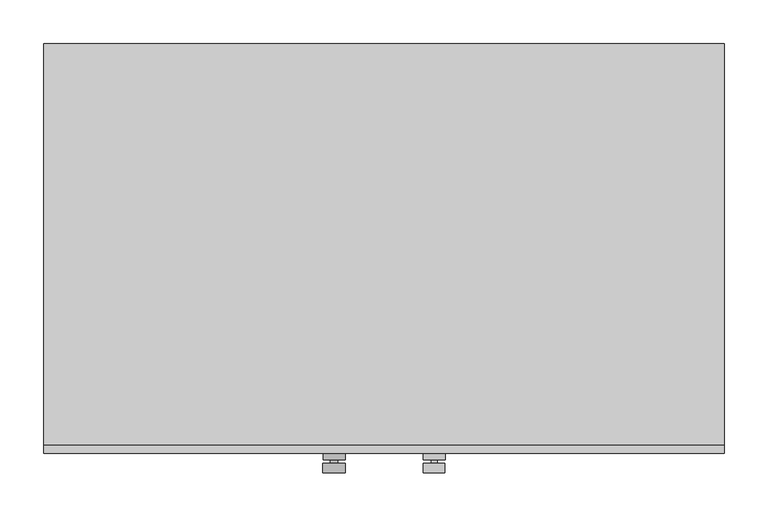
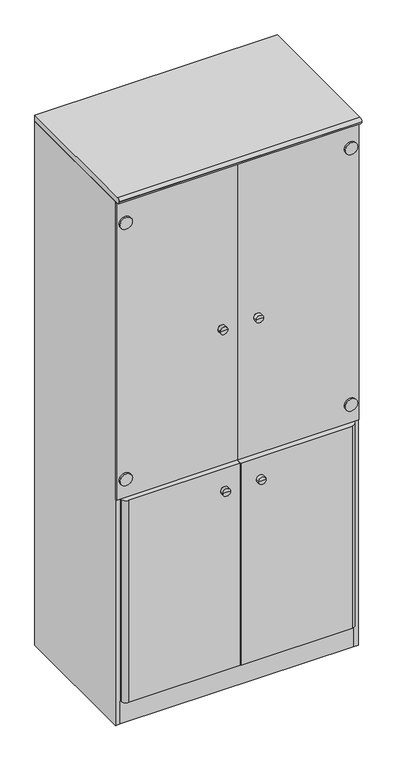
"""IFC4 building model written with IfcOpenShell, lengths in millimetres: furniture geometry, 书柜5 : W780*D450*H1800mm."""

import ifcopenshell
import ifcopenshell.guid

model = None  # the IFC model being written
_history = None  # IfcOwnerHistory: only IFC2X3 demands one
_inside = {}  # id of a spatial element -> (the spatial element, [elements in it])
_under = {}  # id of a project, library or spatial element -> (it, [spatial elements below it])
_declared = {}  # id of a project -> (the project, [libraries it declares])
_typed = {}  # id of a type object -> (the type object, [elements of that type])
_made_of = {}  # id of a material, layer set ... -> (it, [elements and type objects made of it])


def new_model(schema):
    """Start an empty IFC model of exactly this schema.

    Asked for "IFC4X3", IfcOpenShell would pick the latest addendum, in which some entities
    have other attributes; the version numbers below select the first issue.
    IFC2X3 requires an IfcOwnerHistory on every rooted entity: one is made here for all.
    """
    global model, _history
    if schema == "IFC4X3":
        model = ifcopenshell.file(schema_version=(4, 3, 0, 0))
    else:
        model = ifcopenshell.file(schema=schema)
    _inside.clear()
    _under.clear()
    _declared.clear()
    _typed.clear()
    _made_of.clear()
    _history = None
    if model.schema == "IFC2X3":
        org = make("IfcOrganization", Name="unknown")
        user = make(
            "IfcPersonAndOrganization",
            ThePerson=make("IfcPerson", FamilyName="unknown"),
            TheOrganization=org,
        )
        app = make(
            "IfcApplication",
            ApplicationDeveloper=org,
            Version="unknown",
            ApplicationFullName="unknown",
            ApplicationIdentifier="unknown",
        )
        _history = make(
            "IfcOwnerHistory",
            OwningUser=user,
            OwningApplication=app,
            ChangeAction="ADDED",
            CreationDate=0,
        )
    return model


def make(cls, **values):
    """One entity of the class cls with the attributes given. An attribute that is None is left unset."""
    return model.create_entity(
        cls, **{name: value for name, value in values.items() if value is not None}
    )


def rooted(cls, **values):
    """An entity with a GlobalId (a new one), such as an element, a storey or a relation."""
    return make(cls, GlobalId=ifcopenshell.guid.new(), OwnerHistory=_history, **values)


def si_unit(unit_type, name, prefix=None):
    """IfcSIUnit, for example si_unit("LENGTHUNIT", "METRE", prefix="MILLI")."""
    return make("IfcSIUnit", UnitType=unit_type, Prefix=prefix, Name=name)


def assignment(units):
    """IfcUnitAssignment: the units of a project."""
    return None if units is None else make("IfcUnitAssignment", Units=units)


def point(xyz):
    """IfcCartesianPoint."""
    return None if xyz is None else make("IfcCartesianPoint", Coordinates=xyz)


def direction(xyz):
    """IfcDirection."""
    return None if xyz is None else make("IfcDirection", DirectionRatios=xyz)


def frame(location, z_axis=None, x_axis=None):
    """IfcAxis2Placement3D, a coordinate frame: its origin and axes. An axis left out is left unset."""
    return make(
        "IfcAxis2Placement3D",
        Location=point(location),
        Axis=direction(z_axis),
        RefDirection=direction(x_axis),
    )


def frame_2d(location, x_axis=None):
    """IfcAxis2Placement2D, a coordinate frame in the plane: its origin and x axis."""
    return make(
        "IfcAxis2Placement2D", Location=point(location), RefDirection=direction(x_axis)
    )


def origin():
    """The frame at (0, 0, 0) with its axes left unset."""
    return frame((0.0, 0.0, 0.0))


def origin_with_axes():
    """The frame at (0, 0, 0) with the z axis (0, 0, 1) and the x axis (1, 0, 0) written out."""
    return frame((0.0, 0.0, 0.0), z_axis=(0.0, 0.0, 1.0), x_axis=(1.0, 0.0, 0.0))


def place(relative_to, where):
    """IfcLocalPlacement: puts the frame where relative to a parent placement (None: the world)."""
    return make(
        "IfcLocalPlacement", PlacementRelTo=relative_to, RelativePlacement=where
    )


def context(
    kind, dimensions, precision=None, world=None, true_north=None, identifier=None
):
    """IfcGeometricRepresentationContext, for example the 3D "Model" context."""
    return make(
        "IfcGeometricRepresentationContext",
        ContextIdentifier=identifier,
        ContextType=kind,
        CoordinateSpaceDimension=dimensions,
        Precision=precision,
        WorldCoordinateSystem=world,
        TrueNorth=true_north,
    )


def project(units=None, contexts=None):
    """IfcProject with its units and contexts."""
    return rooted(
        "IfcProject",
        Name="project",
        RepresentationContexts=contexts,
        UnitsInContext=assignment(units),
    )


def spatial(cls, under=None, at=None, **own):
    """A site, building, storey or space (cls), placed at a placement, below another one or the project."""
    s = rooted(cls, ObjectPlacement=at, **own)
    if under is not None:
        _under.setdefault(under.id(), (under, []))[1].append(s)
    return s


def polyline(points):
    """IfcPolyline through the points."""
    return make("IfcPolyline", Points=[point(p) for p in points])


def circle_curve(where, radius):
    """IfcCircle in the frame where."""
    return make("IfcCircle", Position=where, Radius=radius)


def trimmed(basis, trim1, trim2, sense, master):
    """IfcTrimmedCurve: the piece of a basis curve between two trims."""
    return make(
        "IfcTrimmedCurve",
        BasisCurve=basis,
        Trim1=trim1,
        Trim2=trim2,
        SenseAgreement=sense,
        MasterRepresentation=master,
    )


def segment(curve, same_sense, transition):
    """IfcCompositeCurveSegment."""
    return make(
        "IfcCompositeCurveSegment",
        Transition=transition,
        SameSense=same_sense,
        ParentCurve=curve,
    )


def composite_curve(segments, self_intersect=None):
    """IfcCompositeCurve: segments joined end to end."""
    return make("IfcCompositeCurve", Segments=segments, SelfIntersect=self_intersect)


def outline(outer, holes=None, kind="AREA"):
    """IfcArbitraryClosedProfileDef: a profile drawn as a closed curve; with holes, ...WithVoids."""
    if holes is None:
        return make("IfcArbitraryClosedProfileDef", ProfileType=kind, OuterCurve=outer)
    return make(
        "IfcArbitraryProfileDefWithVoids",
        ProfileType=kind,
        OuterCurve=outer,
        InnerCurves=holes,
    )


def extrude(swept, where, along, depth):
    """IfcExtrudedAreaSolid: the profile swept, set in the frame where, extruded along a direction by depth."""
    return make(
        "IfcExtrudedAreaSolid",
        SweptArea=swept,
        Position=where,
        ExtrudedDirection=direction(along),
        Depth=depth,
    )


def shape(context_of_items, identifier, shape_type, items):
    """IfcShapeRepresentation: the items that make up one representation, for example the "Body"."""
    return make(
        "IfcShapeRepresentation",
        ContextOfItems=context_of_items,
        RepresentationIdentifier=identifier,
        RepresentationType=shape_type,
        Items=items,
    )


def source(mapping_origin, context_of_items, identifier, shape_type, items):
    """IfcRepresentationMap: a shape defined once, which mapped items show again and again."""
    return make(
        "IfcRepresentationMap",
        MappingOrigin=mapping_origin,
        MappedRepresentation=shape(context_of_items, identifier, shape_type, items),
    )


def transform(
    local_origin,
    x_axis=None,
    y_axis=None,
    z_axis=None,
    scale=None,
    scale2=None,
    scale3=None,
    uniform=True,
):
    """IfcCartesianTransformationOperator3D, or its non-uniform kind. x_axis, y_axis, z_axis: its Axis1, 2, 3."""
    if uniform:
        return make(
            "IfcCartesianTransformationOperator3D",
            Axis1=direction(x_axis),
            Axis2=direction(y_axis),
            LocalOrigin=point(local_origin),
            Scale=scale,
            Axis3=direction(z_axis),
        )
    return make(
        "IfcCartesianTransformationOperator3DnonUniform",
        Axis1=direction(x_axis),
        Axis2=direction(y_axis),
        LocalOrigin=point(local_origin),
        Scale=scale,
        Axis3=direction(z_axis),
        Scale2=scale2,
        Scale3=scale3,
    )


def mapped(mapping_source, mapping_target):
    """IfcMappedItem: shows the shape of a source again, moved by a transform."""
    return make(
        "IfcMappedItem", MappingSource=mapping_source, MappingTarget=mapping_target
    )


def made_of(thing, what):
    """Note that an element or type object is made of a material, layer set ...; save() writes the relation."""
    if what is not None:
        _made_of.setdefault(what.id(), (what, []))[1].append(thing)
    return thing


def element(
    cls,
    number,
    at=None,
    inside=None,
    cuts=None,
    type_object=None,
    material=None,
    context=None,
    identifier="Body",
    shape_type=None,
    held_by="IfcProductDefinitionShape",
    body=None,
    shapes=None,
    **own,
):
    """One element of the class cls, such as IfcWall. Its Tag is "e" and its number.

    at: its placement. inside: the storey or other place that contains it. cuts: it is an
    opening in that element (IfcRelVoidsElement). A single representation is given by context,
    identifier, shape_type and body (its items); several are given by shapes. held_by: the class
    of the entity that holds the representations. save() writes the other relations.
    """
    e = rooted(cls, Tag="e%d" % number, ObjectPlacement=at, **own)
    if body is not None:
        shapes = [shape(context, identifier, shape_type, body)]
    if shapes is not None:
        e.Representation = make(held_by, Representations=shapes)
    if inside is not None:
        _inside.setdefault(inside.id(), (inside, []))[1].append(e)
    if cuts is not None:
        rooted(
            "IfcRelVoidsElement", RelatingBuildingElement=cuts, RelatedOpeningElement=e
        )
    if type_object is not None:
        _typed.setdefault(type_object.id(), (type_object, []))[1].append(e)
    return made_of(e, material)


def aggregate(whole, parts):
    """IfcRelAggregates: a whole, such as a stair, and the parts it consists of."""
    return rooted("IfcRelAggregates", RelatingObject=whole, RelatedObjects=parts)


def save(model, path):
    """Write the relations noted so far, then the file.

    IfcRelAggregates (storeys below a building ...), IfcRelContainedInSpatialStructure (elements
    in a storey), IfcRelDefinesByType, IfcRelAssociatesMaterial and IfcRelDeclares: one each for
    every whole, place, type object, material and project.
    """
    for whole, parts in _under.values():
        aggregate(whole, parts)
    for where, things in _inside.values():
        rooted(
            "IfcRelContainedInSpatialStructure",
            RelatedElements=things,
            RelatingStructure=where,
        )
    for kind, things in _typed.values():
        rooted("IfcRelDefinesByType", RelatedObjects=things, RelatingType=kind)
    for what, things in _made_of.values():
        rooted("IfcRelAssociatesMaterial", RelatedObjects=things, RelatingMaterial=what)
    for by, libraries in _declared.values():
        rooted("IfcRelDeclares", RelatingContext=by, RelatedDefinitions=libraries)
    model.write(path)


def plane_surface(at):
    """IfcPlane: the flat surface through the origin of the frame at, square to its z axis."""
    return make("IfcPlane", Position=at)


def cylinder_surface(at, radius):
    """IfcCylindricalSurface: all points at the distance radius from the z axis of the frame at."""
    return make("IfcCylindricalSurface", Position=at, Radius=radius)


def advanced_brep(points, edges, surfaces, faces):
    """IfcAdvancedBrep: a solid bounded by faces that lie on surfaces and meet in shared edges.

    An edge is (start, end): straight between two places in points (the first is 0);
    or (start, end, curve); or (start, end, curve, False) where it runs against its curve.
    A face is (place in surfaces, loops), or (place, loops, False) where it looks against
    its surface's normal. A loop lists edges by number (the first is 1), with a minus sign
    where the edge is run from its end to its start. The first loop is the outer one.
    """
    corners = [point(p) for p in points]
    vertices = [make("IfcVertexPoint", VertexGeometry=c) for c in corners]
    made = []
    for start, end, *more in edges:
        made.append(
            make(
                "IfcEdgeCurve",
                EdgeStart=vertices[start],
                EdgeEnd=vertices[end],
                EdgeGeometry=more[0] if more else make("IfcPolyline", Points=[corners[start], corners[end]]),
                SameSense=more[1] if len(more) > 1 else True,
            )
        )
    hull = []
    for where, loops, *sense in faces:
        bounds = []
        for j, loop in enumerate(loops):
            ring = [make("IfcOrientedEdge", EdgeElement=made[abs(k) - 1], Orientation=k > 0) for k in loop]
            bounds.append(
                make(
                    "IfcFaceOuterBound" if j == 0 else "IfcFaceBound",
                    Bound=make("IfcEdgeLoop", EdgeList=ring),
                    Orientation=True,
                )
            )
        hull.append(make("IfcAdvancedFace", Bounds=bounds, FaceSurface=surfaces[where], SameSense=sense[0] if sense else True))
    return make("IfcAdvancedBrep", Outer=make("IfcClosedShell", CfsFaces=hull))


def furniture_aa1a75c8(model_context):
    return source(origin(), model_context, "Body", "SolidModel", [
        extrude(outline(composite_curve([segment(polyline([(-246.5557266, 1800.0), (214.2249346, 1800.0), (214.2249346, 1780.00298), (-246.553178, 1780.00298)]), True, "CONTINUOUS"), segment(trimmed(circle_curve(frame_2d((-246.553178, 1789.2248674)), 9.2218874), [point((-246.553178, 1780.00298))], [point((-255.7750654, 1789.2248674))], False, "CARTESIAN"), True, "CONTINUOUS"), segment(polyline([(-255.7750654, 1789.2248674), (-255.7750654, 1790.7806612)]), True, "CONTINUOUS"), segment(trimmed(circle_curve(frame_2d((-246.5557266, 1790.7806612)), 9.2193388), [point((-255.7750654, 1790.7806612))], [point((-246.5557266, 1800.0))], False, "CARTESIAN"), True, "CONTINUOUS")], self_intersect=False)), frame((-390.267589, 0.0, 0.0), z_axis=(1.0, 0.0, 0.0), x_axis=(0.0, 1.0, 0.0)), (0.0, 0.0, 1.0), 780.0),
        extrude(outline(composite_curve([segment(trimmed(circle_curve(frame_2d((832.0298722, 361.9800403)), 20.0), [point((832.0298722, 381.9800403))], [point((832.0298722, 341.9800403))], False, "CARTESIAN"), True, "CONTINUOUS"), segment(trimmed(circle_curve(frame_2d((832.0298722, 361.9800403)), 20.0), [point((832.0298722, 341.9800403))], [point((832.0298722, 381.9800403))], False, "CARTESIAN"), True, "CONTINUOUS")], self_intersect=False)), frame((0.0, -246.5557266, 0.0), z_axis=(0.0, 1.0, 0.0), x_axis=(0.0, 0.0, 1.0)), (0.0, 0.0, 1.0), 5.7806612),
        extrude(outline(composite_curve([segment(trimmed(circle_curve(frame_2d((1702.9701278, 361.9800403)), 20.0), [point((1702.9701278, 381.9800403))], [point((1702.9701278, 341.9800403))], False, "CARTESIAN"), True, "CONTINUOUS"), segment(trimmed(circle_curve(frame_2d((1702.9701278, 361.9800403)), 20.0), [point((1702.9701278, 341.9800403))], [point((1702.9701278, 381.9800403))], False, "CARTESIAN"), True, "CONTINUOUS")], self_intersect=False)), frame((0.0, -246.5557266, 0.0), z_axis=(0.0, 1.0, 0.0), x_axis=(0.0, 0.0, 1.0)), (0.0, 0.0, 1.0), 5.7806612),
        extrude(outline(composite_curve([segment(trimmed(circle_curve(frame_2d((1702.9701278, -362.5152184)), 20.0), [point((1702.9701278, -382.5152184))], [point((1702.9701278, -342.5152184))], False, "CARTESIAN"), True, "CONTINUOUS"), segment(trimmed(circle_curve(frame_2d((1702.9701278, -362.5152184)), 20.0), [point((1702.9701278, -342.5152184))], [point((1702.9701278, -382.5152184))], False, "CARTESIAN"), True, "CONTINUOUS")], self_intersect=False)), frame((0.0, -246.5557266, 0.0), z_axis=(0.0, 1.0, 0.0), x_axis=(0.0, 0.0, 1.0)), (0.0, 0.0, 1.0), 5.7806612),
        extrude(outline(composite_curve([segment(trimmed(circle_curve(frame_2d((832.0298722, -362.5152184)), 20.0), [point((832.0298722, -382.5152184))], [point((832.0298722, -342.5152184))], False, "CARTESIAN"), True, "CONTINUOUS"), segment(trimmed(circle_curve(frame_2d((832.0298722, -362.5152184)), 20.0), [point((832.0298722, -342.5152184))], [point((832.0298722, -382.5152184))], False, "CARTESIAN"), True, "CONTINUOUS")], self_intersect=False)), frame((0.0, -246.5557266, 0.0), z_axis=(0.0, 1.0, 0.0), x_axis=(0.0, 0.0, 1.0)), (0.0, 0.0, 1.0), 5.7806612),
        extrude(outline(composite_curve([segment(polyline([(-375.3567854, -235.7750654), (-1.4459817, -235.7750654), (-1.4459817, -255.7750654), (-359.5899795, -255.7750654)]), True, "CONTINUOUS"), segment(trimmed(circle_curve(frame_2d((-359.5899795, -240.0082595)), 15.7668059), [point((-359.5899795, -255.7750654))], [point((-375.3567854, -240.0082595))], False, "CARTESIAN"), True, "CONTINUOUS"), segment(polyline([(-375.3567854, -240.0082595), (-375.3567854, -235.7750654)]), True, "CONTINUOUS")], self_intersect=False)), frame((0.0, 0.0, 80.0), z_axis=(0.0, 0.0, 1.0), x_axis=(1.0, 0.0, 0.0)), (0.0, 0.0, 1.0), 686.4),
        advanced_brep(
        [(-57.4433336, -240.7750654, 1241.1237815), (-53.4331008, -240.7750654, 1241.1237815), (-61.4535664, -240.7750654, 1241.1237815), (-69.9433336, -263.0203049, 1241.1237815), (-44.9433336, -263.0203049, 1241.1237815), (-57.4433336, -263.0203049, 1241.1237815), (-69.9433336, -251.699089, 1241.1237815), (-44.9433336, -251.699089, 1241.1237815), (-61.4535664, -251.699089, 1241.1237815), (-53.4331008, -251.699089, 1241.1237815)],
        [
            (0, 1),
            (1, 2, circle_curve(frame((-57.4433336, -240.7750654, 1241.1237815), z_axis=(0.0, 1.0, 0.0), x_axis=(1.0, 0.0, 0.0)), 4.0102328)),
            (2, 0),
            (2, 1, circle_curve(frame((-57.4433336, -240.7750654, 1241.1237815), z_axis=(0.0, 1.0, 0.0), x_axis=(1.0, 0.0, 0.0)), 4.0102328)),
            (3, 4, circle_curve(frame((-57.4433336, -263.0203049, 1241.1237815), z_axis=(0.0, -1.0, 0.0), x_axis=(1.0, 0.0, 0.0)), 12.5)),
            (4, 5),
            (5, 3),
            (4, 3, circle_curve(frame((-57.4433336, -263.0203049, 1241.1237815), z_axis=(0.0, -1.0, 0.0), x_axis=(1.0, 0.0, 0.0)), 12.5)),
            (6, 7, circle_curve(frame((-57.4433336, -251.699089, 1241.1237815), z_axis=(0.0, -1.0, 0.0), x_axis=(1.0, 0.0, 0.0)), 12.5)),
            (7, 4),
            (3, 6),
            (7, 6, circle_curve(frame((-57.4433336, -251.699089, 1241.1237815), z_axis=(0.0, -1.0, 0.0), x_axis=(1.0, 0.0, 0.0)), 12.5)),
            (8, 9, circle_curve(frame((-57.4433336, -251.699089, 1241.1237815), z_axis=(0.0, -1.0, 0.0), x_axis=(1.0, 0.0, 0.0)), 4.0102328)),
            (9, 7),
            (6, 8),
            (9, 8, circle_curve(frame((-57.4433336, -251.699089, 1241.1237815), z_axis=(0.0, -1.0, 0.0), x_axis=(1.0, 0.0, 0.0)), 4.0102328)),
            (1, 9),
            (8, 2),
        ],
        [
            plane_surface(frame((-57.4433336, -240.7750654, 1241.1237815), z_axis=(0.0, 1.0, 0.0), x_axis=(1.0, 0.0, 0.0))),
            plane_surface(frame((-57.4433336, -263.0203049, 1241.1237815), z_axis=(0.0, -1.0, 0.0), x_axis=(1.0, 0.0, 0.0))),
            cylinder_surface(frame((-57.4433336, -165.4689088, 1241.1237815), z_axis=(0.0, 1.0, 0.0), x_axis=(1.0, 0.0, 0.0)), 12.5),
            plane_surface(frame((-57.4433336, -251.699089, 1241.1237815), z_axis=(0.0, 1.0, 0.0), x_axis=(1.0, 0.0, 0.0))),
            cylinder_surface(frame((-57.4433336, -165.4689088, 1241.1237815), z_axis=(0.0, 1.0, 0.0), x_axis=(1.0, 0.0, 0.0)), 4.0102328),
        ],
        [
            (0, [[1, 2, 3]]),
            (0, [[-3, 4, -1]]),
            (1, [[5, 6, 7]]),
            (1, [[8, -7, -6]]),
            (2, [[9, 10, -5, 11]]),
            (2, [[12, -11, -8, -10]]),
            (3, [[13, 14, -9, 15]]),
            (3, [[16, -15, -12, -14]]),
            (4, [[-2, 17, -13, 18]]),
            (4, [[-4, -18, -16, -17]]),
        ],
    ),
        advanced_brep(
        [(60.8777058, -251.699089, 1241.1237815), (53.652176, -251.699089, 1241.1237815), (53.652176, -240.7750654, 1241.1237815), (60.8777058, -240.7750654, 1241.1237815), (69.7649409, -251.699089, 1241.1237815), (44.7649409, -251.699089, 1241.1237815), (69.7649409, -263.0203049, 1241.1237815), (44.7649409, -263.0203049, 1241.1237815), (57.2649409, -263.0203049, 1241.1237815), (57.2649409, -240.7750654, 1241.1237815)],
        [
            (0, 1, circle_curve(frame((57.2649409, -251.699089, 1241.1237815), z_axis=(0.0, 1.0, 0.0), x_axis=(-1.0, 0.0, 0.0)), 3.6127649)),
            (1, 2),
            (2, 3, circle_curve(frame((57.2649409, -240.7750654, 1241.1237815), z_axis=(0.0, -1.0, 0.0), x_axis=(-1.0, 0.0, 0.0)), 3.6127649)),
            (3, 0),
            (1, 0, circle_curve(frame((57.2649409, -251.699089, 1241.1237815), z_axis=(0.0, 1.0, 0.0), x_axis=(-1.0, 0.0, 0.0)), 3.6127649)),
            (3, 2, circle_curve(frame((57.2649409, -240.7750654, 1241.1237815), z_axis=(0.0, -1.0, 0.0), x_axis=(-1.0, 0.0, 0.0)), 3.6127649)),
            (4, 5, circle_curve(frame((57.2649409, -251.699089, 1241.1237815), z_axis=(0.0, 1.0, 0.0), x_axis=(-1.0, 0.0, 0.0)), 12.5)),
            (5, 1),
            (0, 4),
            (5, 4, circle_curve(frame((57.2649409, -251.699089, 1241.1237815), z_axis=(0.0, 1.0, 0.0), x_axis=(-1.0, 0.0, 0.0)), 12.5)),
            (6, 7, circle_curve(frame((57.2649409, -263.0203049, 1241.1237815), z_axis=(0.0, 1.0, 0.0), x_axis=(-1.0, 0.0, 0.0)), 12.5)),
            (7, 5),
            (4, 6),
            (7, 6, circle_curve(frame((57.2649409, -263.0203049, 1241.1237815), z_axis=(0.0, 1.0, 0.0), x_axis=(-1.0, 0.0, 0.0)), 12.5)),
            (8, 7),
            (6, 8),
            (2, 9),
            (9, 3),
        ],
        [
            cylinder_surface(frame((57.2649409, -165.4689088, 1241.1237815), z_axis=(0.0, -1.0, 0.0), x_axis=(-1.0, 0.0, 0.0)), 3.6127649),
            plane_surface(frame((57.2649409, -251.699089, 1241.1237815), z_axis=(0.0, 1.0, 0.0), x_axis=(-1.0, 0.0, 0.0))),
            cylinder_surface(frame((57.2649409, -165.4689088, 1241.1237815), z_axis=(0.0, -1.0, 0.0), x_axis=(-1.0, 0.0, 0.0)), 12.5),
            plane_surface(frame((57.2649409, -263.0203049, 1241.1237815), z_axis=(0.0, -1.0, 0.0), x_axis=(-1.0, 0.0, 0.0))),
            plane_surface(frame((57.2649409, -240.7750654, 1241.1237815), z_axis=(0.0, 1.0, 0.0), x_axis=(-1.0, 0.0, 0.0))),
        ],
        [
            (0, [[1, 2, 3, 4]]),
            (0, [[5, -4, 6, -2]]),
            (1, [[7, 8, -1, 9]]),
            (1, [[10, -9, -5, -8]]),
            (2, [[11, 12, -7, 13]]),
            (2, [[14, -13, -10, -12]]),
            (3, [[15, -11, 16]]),
            (3, [[-16, -14, -15]]),
            (4, [[-3, 17, 18]]),
            (4, [[-6, -18, -17]]),
        ],
    ),
        extrude(outline(polyline([(0.9108037, -235.7750654), (389.732411, -235.7750654), (389.732411, -240.7750654), (0.9108037, -240.7750654), (0.9108037, -235.7750654)])), frame((0.0, 0.0, 769.0), z_axis=(0.0, 0.0, 1.0), x_axis=(1.0, 0.0, 0.0)), (0.0, 0.0, 1.0), 1009.0),
        extrude(outline(polyline([(-1.0891963, -235.7750654), (-1.0891963, -240.7750654), (-390.267589, -240.7750654), (-390.267589, -235.7750654), (-1.0891963, -235.7750654)])), frame((0.0, 0.0, 769.0), z_axis=(0.0, 0.0, 1.0), x_axis=(1.0, 0.0, 0.0)), (0.0, 0.0, 1.0), 1009.0),
        extrude(outline(composite_curve([segment(polyline([(374.8216073, -235.7750654), (374.8216073, -240.0082595)]), True, "CONTINUOUS"), segment(trimmed(circle_curve(frame_2d((359.0548014, -240.0082595)), 15.7668059), [point((374.8216073, -240.0082595))], [point((359.0548014, -255.7750654))], False, "CARTESIAN"), True, "CONTINUOUS"), segment(polyline([(359.0548014, -255.7750654), (0.9108037, -255.7750654), (0.9108037, -235.7750654), (374.8216073, -235.7750654)]), True, "CONTINUOUS")], self_intersect=False)), frame((0.0, 0.0, 80.0), z_axis=(0.0, 0.0, 1.0), x_axis=(1.0, 0.0, 0.0)), (0.0, 0.0, 1.0), 686.4),
        extrude(outline(polyline([(374.8216073, -215.6693649), (-375.1783927, -215.6693649), (-375.1783927, 198.2249346), (374.8216073, 198.2249346), (374.8216073, -215.6693649)])), frame((0.0, 0.0, 749.2), z_axis=(0.0, 0.0, 1.0), x_axis=(1.0, 0.0, 0.0)), (0.0, 0.0, 1.0), 17.2),
        extrude(outline(polyline([(374.8216073, 198.2249346), (-375.1783927, 198.2249346), (-375.1783927, 204.2249346), (374.8216073, 204.2249346), (374.8216073, 198.2249346)])), origin_with_axes(), (0.0, 0.0, 1.0), 60.0),
        extrude(outline(polyline([(374.8216073, -215.6693649), (374.8216073, -235.7750654), (-375.1783927, -235.7750654), (-375.1783927, -215.6693649), (374.8216073, -215.6693649)])), origin_with_axes(), (0.0, 0.0, 1.0), 78.0),
        extrude(outline(polyline([(374.8216073, -215.6693649), (-375.1783927, -215.6693649), (-375.1783927, 214.2249346), (374.8216073, 214.2249346), (374.8216073, -215.6693649)])), frame((0.0, 0.0, 60.0), z_axis=(0.0, 0.0, 1.0), x_axis=(1.0, 0.0, 0.0)), (0.0, 0.0, 1.0), 18.0),
        extrude(outline(polyline([(374.8216073, 198.2249346), (-375.1783927, 198.2249346), (-375.1783927, 204.2249346), (374.8216073, 204.2249346), (374.8216073, 198.2249346)])), frame((0.0, 0.0, 78.0), z_axis=(0.0, 0.0, 1.0), x_axis=(1.0, 0.0, 0.0)), (0.0, 0.0, 1.0), 1702.0),
        advanced_brep(
        [(-57.6217263, -255.7750654, 701.1237815), (-53.4331008, -255.7750654, 701.1237815), (-61.8103517, -255.7750654, 701.1237815), (-70.300119, -278.0203049, 701.1237815), (-44.9433336, -278.0203049, 701.1237815), (-57.6217263, -278.0203049, 701.1237815), (-70.300119, -266.699089, 701.1237815), (-44.9433336, -266.699089, 701.1237815), (-61.8103517, -266.699089, 701.1237815), (-53.4331008, -266.699089, 701.1237815)],
        [
            (0, 1),
            (1, 2, circle_curve(frame((-57.6217263, -255.7750654, 701.1237815), z_axis=(0.0, 1.0, 0.0), x_axis=(1.0, 0.0, 0.0)), 4.1886255)),
            (2, 0),
            (2, 1, circle_curve(frame((-57.6217263, -255.7750654, 701.1237815), z_axis=(0.0, 1.0, 0.0), x_axis=(1.0, 0.0, 0.0)), 4.1886255)),
            (3, 4, circle_curve(frame((-57.6217263, -278.0203049, 701.1237815), z_axis=(0.0, -1.0, 0.0), x_axis=(1.0, 0.0, 0.0)), 12.6783927)),
            (4, 5),
            (5, 3),
            (4, 3, circle_curve(frame((-57.6217263, -278.0203049, 701.1237815), z_axis=(0.0, -1.0, 0.0), x_axis=(1.0, 0.0, 0.0)), 12.6783927)),
            (6, 7, circle_curve(frame((-57.6217263, -266.699089, 701.1237815), z_axis=(0.0, -1.0, 0.0), x_axis=(1.0, 0.0, 0.0)), 12.6783927)),
            (7, 4),
            (3, 6),
            (7, 6, circle_curve(frame((-57.6217263, -266.699089, 701.1237815), z_axis=(0.0, -1.0, 0.0), x_axis=(1.0, 0.0, 0.0)), 12.6783927)),
            (8, 9, circle_curve(frame((-57.6217263, -266.699089, 701.1237815), z_axis=(0.0, -1.0, 0.0), x_axis=(1.0, 0.0, 0.0)), 4.1886255)),
            (9, 7),
            (6, 8),
            (9, 8, circle_curve(frame((-57.6217263, -266.699089, 701.1237815), z_axis=(0.0, -1.0, 0.0), x_axis=(1.0, 0.0, 0.0)), 4.1886255)),
            (1, 9),
            (8, 2),
        ],
        [
            plane_surface(frame((-57.6217263, -255.7750654, 701.1237815), z_axis=(0.0, 1.0, 0.0), x_axis=(1.0, 0.0, 0.0))),
            plane_surface(frame((-57.6217263, -278.0203049, 701.1237815), z_axis=(0.0, -1.0, 0.0), x_axis=(1.0, 0.0, 0.0))),
            cylinder_surface(frame((-57.6217263, -180.4689088, 701.1237815), z_axis=(0.0, 1.0, 0.0), x_axis=(1.0, 0.0, 0.0)), 12.6783927),
            plane_surface(frame((-57.6217263, -266.699089, 701.1237815), z_axis=(0.0, 1.0, 0.0), x_axis=(1.0, 0.0, 0.0))),
            cylinder_surface(frame((-57.6217263, -180.4689088, 701.1237815), z_axis=(0.0, 1.0, 0.0), x_axis=(1.0, 0.0, 0.0)), 4.1886255),
        ],
        [
            (0, [[1, 2, 3]]),
            (0, [[-3, 4, -1]]),
            (1, [[5, 6, 7]]),
            (1, [[8, -7, -6]]),
            (2, [[9, 10, -5, 11]]),
            (2, [[12, -11, -8, -10]]),
            (3, [[13, 14, -9, 15]]),
            (3, [[16, -15, -12, -14]]),
            (4, [[-2, 17, -13, 18]]),
            (4, [[-4, -18, -16, -17]]),
        ],
    ),
        advanced_brep(
        [(60.5209204, -266.699089, 701.1237815), (53.652176, -266.699089, 701.1237815), (53.652176, -255.8777654, 701.1237815), (60.5209204, -255.8777654, 701.1237815), (69.4081555, -266.699089, 701.1237815), (44.7649409, -266.699089, 701.1237815), (69.4081555, -278.0203049, 701.1237815), (44.7649409, -278.0203049, 701.1237815), (57.0865482, -278.0203049, 701.1237815), (57.0865482, -255.8777654, 701.1237815)],
        [
            (0, 1, circle_curve(frame((57.0865482, -266.699089, 701.1237815), z_axis=(0.0, 1.0, 0.0), x_axis=(-1.0, 0.0, 0.0)), 3.4343722)),
            (1, 2),
            (2, 3, circle_curve(frame((57.0865482, -255.8777654, 701.1237815), z_axis=(0.0, -1.0, 0.0), x_axis=(-1.0, 0.0, 0.0)), 3.4343722)),
            (3, 0),
            (1, 0, circle_curve(frame((57.0865482, -266.699089, 701.1237815), z_axis=(0.0, 1.0, 0.0), x_axis=(-1.0, 0.0, 0.0)), 3.4343722)),
            (3, 2, circle_curve(frame((57.0865482, -255.8777654, 701.1237815), z_axis=(0.0, -1.0, 0.0), x_axis=(-1.0, 0.0, 0.0)), 3.4343722)),
            (4, 5, circle_curve(frame((57.0865482, -266.699089, 701.1237815), z_axis=(0.0, 1.0, 0.0), x_axis=(-1.0, 0.0, 0.0)), 12.3216073)),
            (5, 1),
            (0, 4),
            (5, 4, circle_curve(frame((57.0865482, -266.699089, 701.1237815), z_axis=(0.0, 1.0, 0.0), x_axis=(-1.0, 0.0, 0.0)), 12.3216073)),
            (6, 7, circle_curve(frame((57.0865482, -278.0203049, 701.1237815), z_axis=(0.0, 1.0, 0.0), x_axis=(-1.0, 0.0, 0.0)), 12.3216073)),
            (7, 5),
            (4, 6),
            (7, 6, circle_curve(frame((57.0865482, -278.0203049, 701.1237815), z_axis=(0.0, 1.0, 0.0), x_axis=(-1.0, 0.0, 0.0)), 12.3216073)),
            (8, 7),
            (6, 8),
            (2, 9),
            (9, 3),
        ],
        [
            cylinder_surface(frame((57.0865482, -180.4689088, 701.1237815), z_axis=(0.0, -1.0, 0.0), x_axis=(-1.0, 0.0, 0.0)), 3.4343722),
            plane_surface(frame((57.0865482, -266.699089, 701.1237815), z_axis=(0.0, 1.0, 0.0), x_axis=(-1.0, 0.0, 0.0))),
            cylinder_surface(frame((57.0865482, -180.4689088, 701.1237815), z_axis=(0.0, -1.0, 0.0), x_axis=(-1.0, 0.0, 0.0)), 12.3216073),
            plane_surface(frame((57.0865482, -278.0203049, 701.1237815), z_axis=(0.0, -1.0, 0.0), x_axis=(-1.0, 0.0, 0.0))),
            plane_surface(frame((57.0865482, -255.8777654, 701.1237815), z_axis=(0.0, 1.0, 0.0), x_axis=(-1.0, 0.0, 0.0))),
        ],
        [
            (0, [[1, 2, 3, 4]]),
            (0, [[5, -4, 6, -2]]),
            (1, [[7, 8, -1, 9]]),
            (1, [[10, -9, -5, -8]]),
            (2, [[11, 12, -7, 13]]),
            (2, [[14, -13, -10, -12]]),
            (3, [[15, -11, 16]]),
            (3, [[-16, -14, -15]]),
            (4, [[-3, 17, 18]]),
            (4, [[-6, -18, -17]]),
        ],
    ),
        extrude(outline(polyline([(374.8216073, 198.2249346), (374.8216073, -215.6693649), (-375.1783927, -215.6693649), (-375.1783927, 198.2249346), (374.8216073, 198.2249346)])), frame((0.0, 0.0, 1095.2666667), z_axis=(0.0, 0.0, 1.0), x_axis=(1.0, 0.0, 0.0)), (0.0, 0.0, 1.0), 18.0),
        extrude(outline(polyline([(374.8216073, 198.2249346), (374.8216073, -215.6693649), (-375.1783927, -215.6693649), (-375.1783927, 198.2249346), (374.8216073, 198.2249346)])), frame((0.0, 0.0, 1433.1333333), z_axis=(0.0, 0.0, 1.0), x_axis=(1.0, 0.0, 0.0)), (0.0, 0.0, 1.0), 18.0),
        extrude(outline(polyline([(-390.267589, 214.2249346), (-375.1783927, 214.2249346), (-375.1783927, -235.7750654), (-390.267589, -235.7750654), (-390.267589, 214.2249346)])), origin_with_axes(), (0.0, 0.0, 1.0), 1780.0),
        extrude(outline(polyline([(389.732411, 214.2249346), (389.732411, -235.7750654), (374.8216073, -235.7750654), (374.8216073, 214.2249346), (389.732411, 214.2249346)])), origin_with_axes(), (0.0, 0.0, 1.0), 1780.0),
    ])


if __name__ == "__main__":
    model = new_model("IFC4")
    model_context = context("Model", 3, world=origin())
    ifc_project = project(units=[si_unit("LENGTHUNIT", "METRE", prefix="MILLI")], contexts=[model_context])
    site = spatial("IfcSite", under=ifc_project)
    building = spatial("IfcBuilding", under=site)
    placement = place(None, origin())
    furniture_shape = furniture_aa1a75c8(model_context)
    element("IfcFurniture", 1, ObjectType="书柜5 : W780*D450*H1800mm", at=placement, inside=building, context=model_context, shape_type="MappedRepresentation", body=[
        mapped(furniture_shape, transform((0.0, 0.0, 0.0), x_axis=(1.0, 0.0, 0.0), y_axis=(0.0, 1.0, 0.0), z_axis=(0.0, 0.0, 1.0))),
    ])
    save(model, "model.ifc")

# Revit data of these elements
# Type "书柜5 : W780*D450*H1800mm"
#   W = 780 mm
#   H = 1800 mm
#   D = 450 mm
#   门板材质 = 木质面层(1)
#   搁板材质 = 白油漆
#   配件材质 = 金属 - 不锈钢，抛光
#   玻璃材质 = 玻璃
#   Manufacturer = ""
#   Model = ""
# Element 1 (IfcFurniture, "书柜5 : W780*D450*H1800mm")
#   Materials on its faces: "木质面层(1)", "金属 - 不锈钢，抛光", "白油漆", "玻璃"
# Materials
#   "木质面层(1)": class "木质", colour RGB 173 104 78, transparency 0
#   "白油漆": class "油漆", colour RGB 252 252 252, transparency 0
#   "金属 - 不锈钢，抛光": class "金属", colour RGB 236 239 239, transparency 0, Cost = 0
#   "玻璃": class "玻璃", colour RGB 0 128 192, transparency 0.9, Description = "钠钙玻璃", Cost = 0
